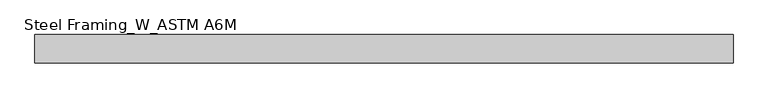
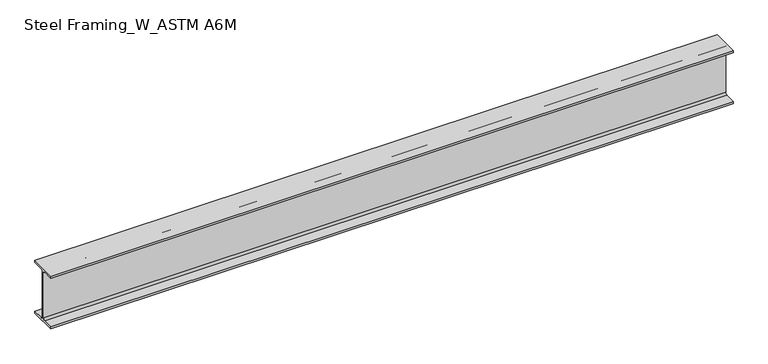
"""IFC4 building model written with IfcOpenShell, lengths in millimetres: beam geometry, Steel Framing_W_ASTM A6M : H_SB_AR_S02_W200x22.5_J1."""

from ifc_helpers import new_model, si_unit, point, frame, frame_2d, origin, place, context, project, spatial, polyline, circle_curve, trimmed, segment, composite_curve, outline, extrude, source, transform, mapped, element, save


def steel_framing_w_astm_a6m_0cfad42d(model_context):
    return source(origin(), model_context, "Body", "SweptSolid", [
        extrude(outline(composite_curve([segment(polyline([(51.0, -95.0), (51.0, -103.0), (-51.0, -103.0), (-51.0, -95.0), (-10.71, -95.0)]), True, "CONTINUOUS"), segment(trimmed(circle_curve(frame_2d((-10.71, -87.4)), 7.6), [point((-10.71, -95.0))], [point((-3.11, -87.4))], True, "CARTESIAN"), True, "CONTINUOUS"), segment(polyline([(-3.11, -87.4), (-3.11, 87.4)]), True, "CONTINUOUS"), segment(trimmed(circle_curve(frame_2d((-10.71, 87.4)), 7.6), [point((-3.11, 87.4))], [point((-10.71, 95.0))], True, "CARTESIAN"), True, "CONTINUOUS"), segment(polyline([(-10.71, 95.0), (-51.0, 95.0), (-51.0, 103.0), (51.0, 103.0), (51.0, 95.0), (10.71, 95.0)]), True, "CONTINUOUS"), segment(trimmed(circle_curve(frame_2d((10.71, 87.4)), 7.6), [point((10.71, 95.0))], [point((3.11, 87.4))], True, "CARTESIAN"), True, "CONTINUOUS"), segment(polyline([(3.11, 87.4), (3.11, -87.4)]), True, "CONTINUOUS"), segment(trimmed(circle_curve(frame_2d((10.71, -87.4)), 7.6), [point((3.11, -87.4))], [point((10.71, -95.0))], True, "CARTESIAN"), True, "CONTINUOUS"), segment(polyline([(10.71, -95.0), (51.0, -95.0)]), True, "CONTINUOUS")], self_intersect=False)), frame((-1195.3, 0.0, 0.0), z_axis=(1.0, 0.0, 0.0), x_axis=(0.0, 1.0, 0.0)), (0.0, 0.0, 1.0), 2517.5),
    ])


if __name__ == "__main__":
    model = new_model("IFC4")
    model_context = context("Model", 3, world=origin())
    ifc_project = project(units=[si_unit("LENGTHUNIT", "METRE", prefix="MILLI")], contexts=[model_context])
    site = spatial("IfcSite", under=ifc_project)
    building = spatial("IfcBuilding", under=site)
    placement = place(None, origin())
    steel_framing_w_astm_a6m_shape = steel_framing_w_astm_a6m_0cfad42d(model_context)
    element("IfcBeam", 1, ObjectType="Steel Framing_W_ASTM A6M : H_SB_AR_S02_W200x22.5_J1", at=placement, inside=building, context=model_context, shape_type="MappedRepresentation", body=[
        mapped(steel_framing_w_astm_a6m_shape, transform((0.0, 0.0, 0.0), x_axis=(1.0, 0.0, 0.0), y_axis=(0.0, 1.0, 0.0), z_axis=(0.0, 0.0, 1.0))),
    ])
    save(model, "model.ifc")

# Revit data of these elements
# Type "Steel Framing_W_ASTM A6M : H_SB_AR_S02_W200x22.5_J1"
#   Section Name Key = "W8x15"
#   Width = 10.2 cm
#   Web Thickness = 0.622 cm
#   Web Fillet = 0.76 cm
#   Warping Constant = 13900.0 cm⁶
#   Torsional Moment of Inertia = 5.70 cm⁴
#   Section Area = 28.6 cm²
#   Plastic Modulus weak axis = 43.8 cm³
#   Plastic Modulus strong axis = 223.0 cm³
#   Perimeter = 0.795 m²/m
#   Nominal Weight = 22.50 kgf/m
#   Moment of Inertia weak axis = 142.00 cm⁴
#   Moment of Inertia strong axis = 2000.00 cm⁴
#   Height = 20.6 cm
#   Flange Thickness = 0.8 cm
#   Elastic Modulus weak axis = 27.9 cm³
#   Elastic Modulus strong axis = 193.0 cm³
#   Centroid Vertical = 10.3 cm
#   Centroid Horizontal = 5.1 cm
#   Length [instance default] = 1500 mm
#   Structural Material [instance default] = Steel, 45-345
#   Bolt Spacing = 0
#   Assembly Code = ""
# Element 1 (IfcBeam, "Steel Framing_W_ASTM A6M : H_SB_AR_S02_W200x22.5_J1")
#   Materials on its faces: "Steel, 45-345"
# Materials
#   "Steel, 45-345": class "Metal", colour RGB 189 187 185, transparency 0, Description = "Steel 345 MPa", Cost = 0
